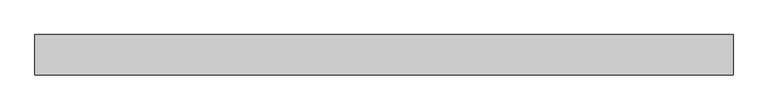
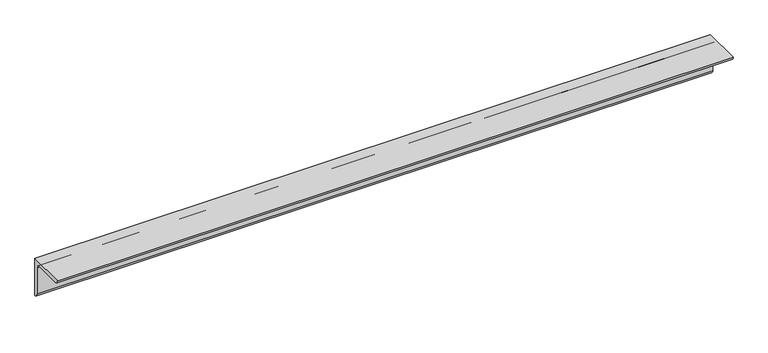
"""IFC4 building model written with IfcOpenShell, lengths in millimetres: beam geometry, 0912_Steel Framing_L-KSD3502 : H_SB_AR_S04_L-100x100x10_KBR2."""

from ifc_helpers import new_model, si_unit, point, frame, frame_2d, origin, place, context, project, spatial, polyline, circle_curve, trimmed, segment, composite_curve, outline, extrude, source, transform, mapped, element, save


def beam_7f428fab(model_context):
    return source(origin(), model_context, "Body", "SweptSolid", [
        extrude(outline(composite_curve([segment(polyline([(28.2, 28.2), (28.2, -71.8)]), True, "CONTINUOUS"), segment(trimmed(circle_curve(frame_2d((28.2, -61.8)), 10.0), [point((28.2, -71.8))], [point((18.2, -61.8))], False, "CARTESIAN"), True, "CONTINUOUS"), segment(polyline([(18.2, -61.8), (18.2, 8.2)]), True, "CONTINUOUS"), segment(trimmed(circle_curve(frame_2d((8.2, 8.2)), 10.0), [point((18.2, 8.2))], [point((8.2, 18.2))], True, "CARTESIAN"), True, "CONTINUOUS"), segment(polyline([(8.2, 18.2), (-61.8, 18.2)]), True, "CONTINUOUS"), segment(trimmed(circle_curve(frame_2d((-61.8, 28.2)), 10.0), [point((-61.8, 18.2))], [point((-71.8, 28.2))], False, "CARTESIAN"), True, "CONTINUOUS"), segment(polyline([(-71.8, 28.2), (28.2, 28.2)]), True, "CONTINUOUS")], self_intersect=False)), frame((-853.0825032, 0.0, 0.0), z_axis=(1.0, 0.0, 0.0), x_axis=(0.0, 1.0, 0.0)), (0.0, 0.0, 1.0), 1723.8034376),
    ])


if __name__ == "__main__":
    model = new_model("IFC4")
    model_context = context("Model", 3, world=origin())
    ifc_project = project(units=[si_unit("LENGTHUNIT", "METRE", prefix="MILLI")], contexts=[model_context])
    site = spatial("IfcSite", under=ifc_project)
    building = spatial("IfcBuilding", under=site)
    placement = place(None, origin())
    beam_shape = beam_7f428fab(model_context)
    element("IfcBeam", 1, ObjectType="0912_Steel Framing_L-KSD3502 : H_SB_AR_S04_L-100x100x10_KBR2", at=placement, inside=building, context=model_context, shape_type="MappedRepresentation", body=[
        mapped(beam_shape, transform((0.0, 0.0, 0.0), x_axis=(1.0, 0.0, 0.0), y_axis=(0.0, 1.0, 0.0), z_axis=(0.0, 0.0, 1.0))),
    ])
    save(model, "model.ifc")

# Revit data of these elements
# Type "0912_Steel Framing_L-KSD3502 : H_SB_AR_S04_L-100x100x10_KBR2"
#   k = 25 mm
#   Perimeter = 0.40 m²/m
#   Nominal Weight = 14.90 kgf/m
#   Length [instance default] = 1000 mm
#   b = 100 mm
#   d = 100 mm
#   t = 10 mm
#   x = 28.2 mm
#   y = 28.2 mm
#   A = 1900.00 m²
#   Structural Material [instance default] = Steel, 45-345
# Element 1 (IfcBeam, "0912_Steel Framing_L-KSD3502 : H_SB_AR_S04_L-100x100x10_KBR2")
#   Structural Material = Steel ASTM A36
#   Materials on its faces: "Steel ASTM A36"
# Materials
#   "Steel, 45-345": class "Metal", colour RGB 189 187 185, transparency 0, Description = "Steel 345 MPa", Cost = 0
#   "Steel ASTM A36": class "Metal", colour RGB 199 199 199, transparency 0, Description = "Structural steel, ASTM A36 Grade B, mill finish", Cost = 0
